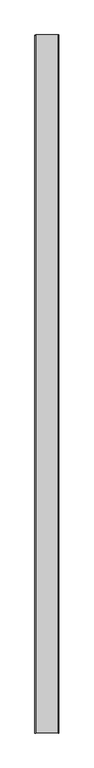
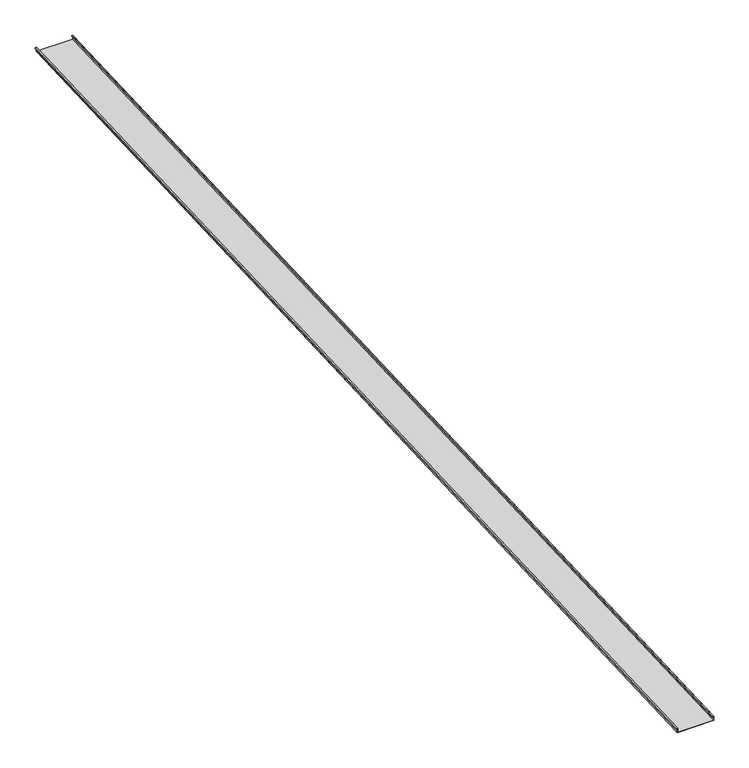
"""IFC4 building model written with IfcOpenShell, lengths in millimetres: proxy geometry, Generic Models 2:Generic Models 2:310765:Generic Models 2:310765 : Generic Models 2:Generic Models 2:310765:14 : Generic Models 2:Generic Models 2:310765:Generic Models 2:310765 : Generic Models 2:Generic Models 2:310765:300385."""

from ifc_helpers import new_model, si_unit, frame, origin, place, context, project, spatial, polyline, outline, extrude, source, transform, mapped, element, save


def generic_models_5ff6fe73(model_context):
    return source(origin(), model_context, "Body", "SweptSolid", [
        extrude(outline(polyline([(1.5875, 0.0), (1.5875, 50.8), (407.9875, 50.8), (407.9875, 1.5874999), (396.875, 1.5874999), (396.875, 11.1124999), (398.4625, 11.1124999), (398.4625, 3.175), (406.4, 3.175), (406.4, 49.2124999), (3.175, 49.2124999), (3.175, -1.5875), (-14.2875, -1.5875), (-14.2875, 9.525), (-12.7, 9.525), (-12.7, 0.0), (1.5875, 0.0)])), frame((592719.1763073, -580680.1387482, 3930.765456), z_axis=(0.0, 0.9991330730923568, 0.04163054471206784), x_axis=(1.0, 0.0, 0.0)), (0.0, 0.0, 1.0), 12437.8358634),
    ])


if __name__ == "__main__":
    model = new_model("IFC4")
    model_context = context("Model", 3, world=origin())
    ifc_project = project(units=[si_unit("LENGTHUNIT", "METRE", prefix="MILLI")], contexts=[model_context])
    site = spatial("IfcSite", under=ifc_project)
    building = spatial("IfcBuilding", under=site)
    placement = place(None, origin())
    generic_models_shape = generic_models_5ff6fe73(model_context)
    element("IfcBuildingElementProxy", 1, Name="Generic Models 2:Generic Models 2:310765:Generic Models 2:310765 : Generic Models 2:Generic Models 2:310765:14 : Generic Models 2:Generic Models 2:310765:Generic Models 2:310765 : Generic Models 2:Generic Models 2:310765:300385", ObjectType="Generic Models 2:Generic Models 2:310765:Generic Models 2:310765 : Generic Models 2:Generic Models 2:310765:14 : Generic Models 2:Generic Models 2:310765:Generic Models 2:310765 : Generic Models 2:Generic Models 2:310765:300385", at=placement, inside=building, context=model_context, shape_type="MappedRepresentation", body=[
        mapped(generic_models_shape, transform((0.0, 0.0, 0.0), x_axis=(1.0, 0.0, 0.0), y_axis=(0.0, 1.0, 0.0), z_axis=(0.0, 0.0, 1.0))),
    ])
    save(model, "model.ifc")

# Revit data of these elements
# Type "Generic Models 2:Generic Models 2:310765:Generic Models 2:310765 : Generic Models 2:Generic Models 2:310765:14 : Generic Models 2:Generic Models 2:310765:Generic Models 2:310765 : Generic Models 2:Generic Models 2:310765:300385"
#   NameOverride = "Generic Models 2:Generic Models 2:310765:Generic Models 2:310765 : Generic Models 2:Generic Models 2:310765:300385"
#   ObjectTypeOverride = "Generic Models 2:310765 : Generic Models 2:Generic Models 2:310765"
#   Reference = "Generic Models 2"
#   Tag = "300385"
# Element 1 (IfcBuildingElementProxy, "Generic Models 2:Generic Models 2:310765:Generic Models 2:310765 : Generic Models 2:Generic Models 2:310765:14 : Generic Models 2:Generic Models 2:310765:Generic Models 2:310765 : Generic Models 2:Generic Models 2:310765:300385")
#   Materials on its faces: "STRUCTURAL STANDING SEAM SHEET METAL ROOFING - BATTENLOK - COLOR T.B.D."
# Materials
#   "STRUCTURAL STANDING SEAM SHEET METAL ROOFING - BATTENLOK - COLOR T.B.D.": class "Generic", colour RGB 120 120 120, transparency 0, Cost = 0
